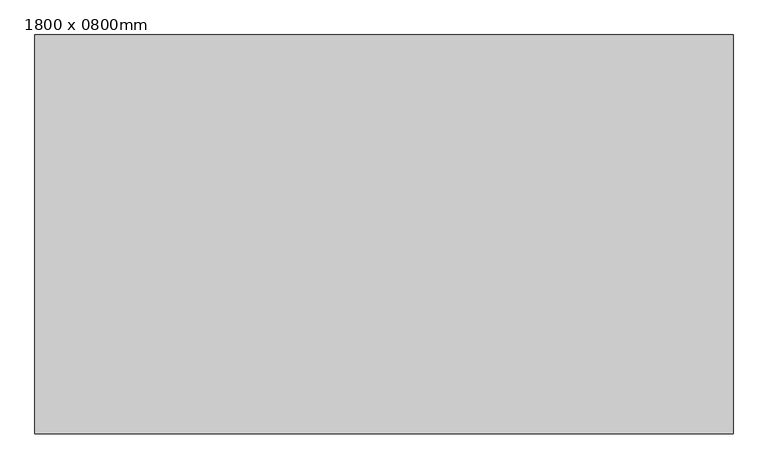
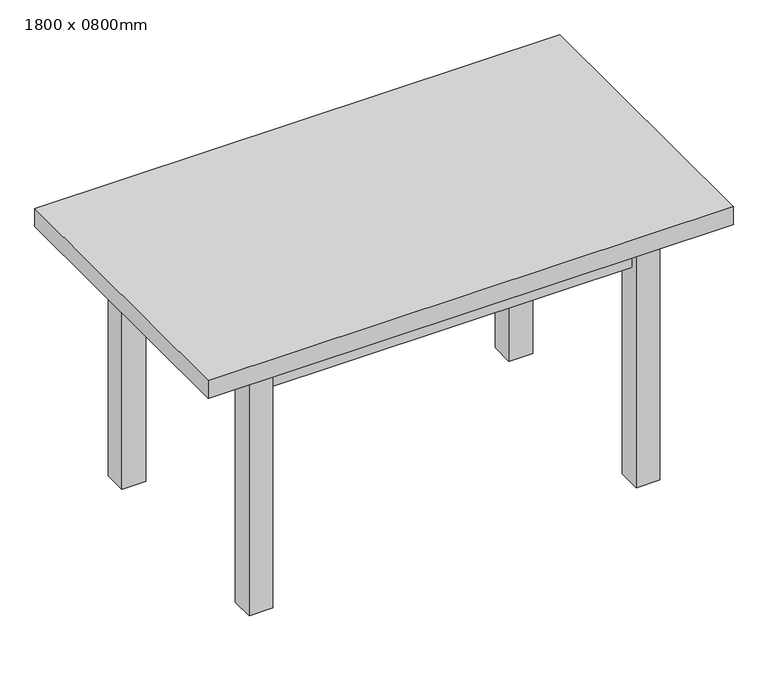
"""IFC4 building model written with IfcOpenShell, lengths in millimetres: furniture geometry, Mesa-Retangular.rfaddd : 1800 x 0800mm."""

from ifc_helpers import new_model, si_unit, frame, origin, origin_with_axes, place, context, project, spatial, polyline, outline, extrude, source, transform, mapped, element, save


def furniture_1800_x_0800mm_c1e0a97f(model_context):
    return source(origin(), model_context, "Body", "SweptSolid", [
        extrude(outline(polyline([(522.2, 305.8060421), (522.2, -305.8060421), (-522.2, -305.8060421), (-522.2, 305.8060421), (522.2, 305.8060421)]), holes=[polyline([(496.8, 253.5139786), (-496.8, 253.5139786), (-496.8, -219.4131933), (496.8, -219.4131933), (496.8, 253.5139786)])]), frame((0.0, 0.0, 609.6), z_axis=(0.0, 0.0, 1.0), x_axis=(1.0, 0.0, 0.0)), (0.0, 0.0, 1.0), 101.6),
        extrude(outline(polyline([(700.0, 400.0), (700.0, -400.0), (-700.0, -400.0), (-700.0, 400.0), (700.0, 400.0)])), frame((0.0, 0.0, 711.2), z_axis=(0.0, 0.0, 1.0), x_axis=(1.0, 0.0, 0.0)), (0.0, 0.0, 1.0), 50.8),
        extrude(outline(polyline([(-484.1, 325.6), (-484.1, 262.1), (-547.6, 262.1), (-547.6, 325.6), (-484.1, 325.6)])), origin_with_axes(), (0.0, 0.0, 1.0), 711.2),
        extrude(outline(polyline([(484.1, 325.6), (547.6, 325.6), (547.6, 262.1), (484.1, 262.1), (484.1, 325.6)])), origin_with_axes(), (0.0, 0.0, 1.0), 711.2),
        extrude(outline(polyline([(-484.1, -325.6), (-547.6, -325.6), (-547.6, -262.1), (-484.1, -262.1), (-484.1, -325.6)])), origin_with_axes(), (0.0, 0.0, 1.0), 711.2),
        extrude(outline(polyline([(484.1, -325.6), (484.1, -262.1), (547.6, -262.1), (547.6, -325.6), (484.1, -325.6)])), origin_with_axes(), (0.0, 0.0, 1.0), 711.2),
    ])


if __name__ == "__main__":
    model = new_model("IFC4")
    model_context = context("Model", 3, world=origin())
    ifc_project = project(units=[si_unit("LENGTHUNIT", "METRE", prefix="MILLI")], contexts=[model_context])
    site = spatial("IfcSite", under=ifc_project)
    building = spatial("IfcBuilding", under=site)
    placement = place(None, origin())
    furniture_1800_x_0800mm_shape = furniture_1800_x_0800mm_c1e0a97f(model_context)
    element("IfcFurniture", 1, ObjectType="Mesa-Retangular.rfaddd : 1800 x 0800mm", at=placement, inside=building, context=model_context, shape_type="MappedRepresentation", body=[
        mapped(furniture_1800_x_0800mm_shape, transform((0.0, 0.0, 0.0), x_axis=(1.0, 0.0, 0.0), y_axis=(0.0, 1.0, 0.0), z_axis=(0.0, 0.0, 1.0))),
    ])
    save(model, "model.ifc")

# Revit data of these elements
# Type "Mesa-Retangular.rfaddd : 1800 x 0800mm"
#   Altura = 0.762 m
#   Comprimento = 1.4 m
#   Largura = 0.8 m
#   Material base = Wood Cherry
#   Material superior = Wood Cherry
#   Default Elevation = 0
# Element 1 (IfcFurniture, "Mesa-Retangular.rfaddd : 1800 x 0800mm")
#   Materials on its faces: "Wood Cherry"
# Materials
#   "Wood Cherry": class "Unassigned", colour RGB 185 153 118, transparency 0
